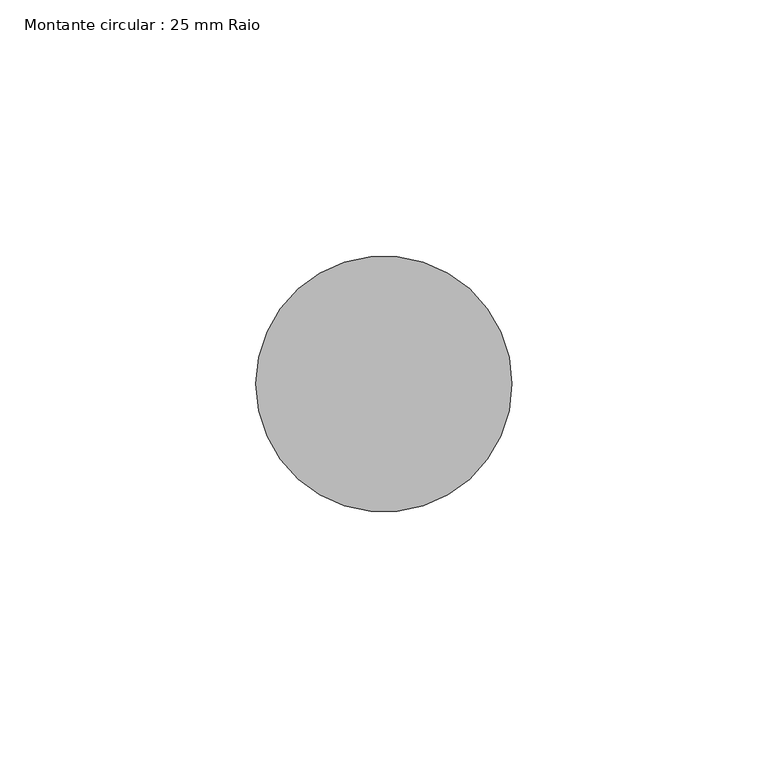
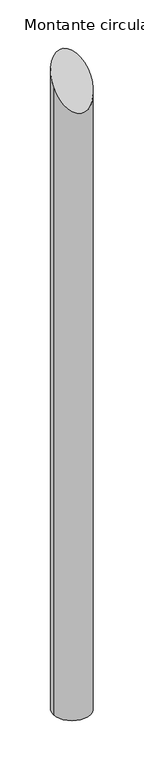
"""IFC4 building model written with IfcOpenShell, lengths in millimetres: member geometry, Montante circular : 25 mm Raio."""

import ifcopenshell
import ifcopenshell.guid

model = None  # the IFC model being written
_history = None  # IfcOwnerHistory: only IFC2X3 demands one
_inside = {}  # id of a spatial element -> (the spatial element, [elements in it])
_under = {}  # id of a project, library or spatial element -> (it, [spatial elements below it])
_declared = {}  # id of a project -> (the project, [libraries it declares])
_typed = {}  # id of a type object -> (the type object, [elements of that type])
_made_of = {}  # id of a material, layer set ... -> (it, [elements and type objects made of it])


def new_model(schema):
    """Start an empty IFC model of exactly this schema.

    Asked for "IFC4X3", IfcOpenShell would pick the latest addendum, in which some entities
    have other attributes; the version numbers below select the first issue.
    IFC2X3 requires an IfcOwnerHistory on every rooted entity: one is made here for all.
    """
    global model, _history
    if schema == "IFC4X3":
        model = ifcopenshell.file(schema_version=(4, 3, 0, 0))
    else:
        model = ifcopenshell.file(schema=schema)
    _inside.clear()
    _under.clear()
    _declared.clear()
    _typed.clear()
    _made_of.clear()
    _history = None
    if model.schema == "IFC2X3":
        org = make("IfcOrganization", Name="unknown")
        user = make(
            "IfcPersonAndOrganization",
            ThePerson=make("IfcPerson", FamilyName="unknown"),
            TheOrganization=org,
        )
        app = make(
            "IfcApplication",
            ApplicationDeveloper=org,
            Version="unknown",
            ApplicationFullName="unknown",
            ApplicationIdentifier="unknown",
        )
        _history = make(
            "IfcOwnerHistory",
            OwningUser=user,
            OwningApplication=app,
            ChangeAction="ADDED",
            CreationDate=0,
        )
    return model


def make(cls, **values):
    """One entity of the class cls with the attributes given. An attribute that is None is left unset."""
    return model.create_entity(
        cls, **{name: value for name, value in values.items() if value is not None}
    )


def rooted(cls, **values):
    """An entity with a GlobalId (a new one), such as an element, a storey or a relation."""
    return make(cls, GlobalId=ifcopenshell.guid.new(), OwnerHistory=_history, **values)


def si_unit(unit_type, name, prefix=None):
    """IfcSIUnit, for example si_unit("LENGTHUNIT", "METRE", prefix="MILLI")."""
    return make("IfcSIUnit", UnitType=unit_type, Prefix=prefix, Name=name)


def assignment(units):
    """IfcUnitAssignment: the units of a project."""
    return None if units is None else make("IfcUnitAssignment", Units=units)


def point(xyz):
    """IfcCartesianPoint."""
    return None if xyz is None else make("IfcCartesianPoint", Coordinates=xyz)


def direction(xyz):
    """IfcDirection."""
    return None if xyz is None else make("IfcDirection", DirectionRatios=xyz)


def frame(location, z_axis=None, x_axis=None):
    """IfcAxis2Placement3D, a coordinate frame: its origin and axes. An axis left out is left unset."""
    return make(
        "IfcAxis2Placement3D",
        Location=point(location),
        Axis=direction(z_axis),
        RefDirection=direction(x_axis),
    )


def origin():
    """The frame at (0, 0, 0) with its axes left unset."""
    return frame((0.0, 0.0, 0.0))


def place(relative_to, where):
    """IfcLocalPlacement: puts the frame where relative to a parent placement (None: the world)."""
    return make(
        "IfcLocalPlacement", PlacementRelTo=relative_to, RelativePlacement=where
    )


def context(
    kind, dimensions, precision=None, world=None, true_north=None, identifier=None
):
    """IfcGeometricRepresentationContext, for example the 3D "Model" context."""
    return make(
        "IfcGeometricRepresentationContext",
        ContextIdentifier=identifier,
        ContextType=kind,
        CoordinateSpaceDimension=dimensions,
        Precision=precision,
        WorldCoordinateSystem=world,
        TrueNorth=true_north,
    )


def project(units=None, contexts=None):
    """IfcProject with its units and contexts."""
    return rooted(
        "IfcProject",
        Name="project",
        RepresentationContexts=contexts,
        UnitsInContext=assignment(units),
    )


def spatial(cls, under=None, at=None, **own):
    """A site, building, storey or space (cls), placed at a placement, below another one or the project."""
    s = rooted(cls, ObjectPlacement=at, **own)
    if under is not None:
        _under.setdefault(under.id(), (under, []))[1].append(s)
    return s


def circle_curve(where, radius):
    """IfcCircle in the frame where."""
    return make("IfcCircle", Position=where, Radius=radius)


def ellipse_curve(where, semi_axis1, semi_axis2):
    """IfcEllipse in the frame where."""
    return make(
        "IfcEllipse", Position=where, SemiAxis1=semi_axis1, SemiAxis2=semi_axis2
    )


def shape(context_of_items, identifier, shape_type, items):
    """IfcShapeRepresentation: the items that make up one representation, for example the "Body"."""
    return make(
        "IfcShapeRepresentation",
        ContextOfItems=context_of_items,
        RepresentationIdentifier=identifier,
        RepresentationType=shape_type,
        Items=items,
    )


def source(mapping_origin, context_of_items, identifier, shape_type, items):
    """IfcRepresentationMap: a shape defined once, which mapped items show again and again."""
    return make(
        "IfcRepresentationMap",
        MappingOrigin=mapping_origin,
        MappedRepresentation=shape(context_of_items, identifier, shape_type, items),
    )


def transform(
    local_origin,
    x_axis=None,
    y_axis=None,
    z_axis=None,
    scale=None,
    scale2=None,
    scale3=None,
    uniform=True,
):
    """IfcCartesianTransformationOperator3D, or its non-uniform kind. x_axis, y_axis, z_axis: its Axis1, 2, 3."""
    if uniform:
        return make(
            "IfcCartesianTransformationOperator3D",
            Axis1=direction(x_axis),
            Axis2=direction(y_axis),
            LocalOrigin=point(local_origin),
            Scale=scale,
            Axis3=direction(z_axis),
        )
    return make(
        "IfcCartesianTransformationOperator3DnonUniform",
        Axis1=direction(x_axis),
        Axis2=direction(y_axis),
        LocalOrigin=point(local_origin),
        Scale=scale,
        Axis3=direction(z_axis),
        Scale2=scale2,
        Scale3=scale3,
    )


def mapped(mapping_source, mapping_target):
    """IfcMappedItem: shows the shape of a source again, moved by a transform."""
    return make(
        "IfcMappedItem", MappingSource=mapping_source, MappingTarget=mapping_target
    )


def made_of(thing, what):
    """Note that an element or type object is made of a material, layer set ...; save() writes the relation."""
    if what is not None:
        _made_of.setdefault(what.id(), (what, []))[1].append(thing)
    return thing


def element(
    cls,
    number,
    at=None,
    inside=None,
    cuts=None,
    type_object=None,
    material=None,
    context=None,
    identifier="Body",
    shape_type=None,
    held_by="IfcProductDefinitionShape",
    body=None,
    shapes=None,
    **own,
):
    """One element of the class cls, such as IfcWall. Its Tag is "e" and its number.

    at: its placement. inside: the storey or other place that contains it. cuts: it is an
    opening in that element (IfcRelVoidsElement). A single representation is given by context,
    identifier, shape_type and body (its items); several are given by shapes. held_by: the class
    of the entity that holds the representations. save() writes the other relations.
    """
    e = rooted(cls, Tag="e%d" % number, ObjectPlacement=at, **own)
    if body is not None:
        shapes = [shape(context, identifier, shape_type, body)]
    if shapes is not None:
        e.Representation = make(held_by, Representations=shapes)
    if inside is not None:
        _inside.setdefault(inside.id(), (inside, []))[1].append(e)
    if cuts is not None:
        rooted(
            "IfcRelVoidsElement", RelatingBuildingElement=cuts, RelatedOpeningElement=e
        )
    if type_object is not None:
        _typed.setdefault(type_object.id(), (type_object, []))[1].append(e)
    return made_of(e, material)


def aggregate(whole, parts):
    """IfcRelAggregates: a whole, such as a stair, and the parts it consists of."""
    return rooted("IfcRelAggregates", RelatingObject=whole, RelatedObjects=parts)


def save(model, path):
    """Write the relations noted so far, then the file.

    IfcRelAggregates (storeys below a building ...), IfcRelContainedInSpatialStructure (elements
    in a storey), IfcRelDefinesByType, IfcRelAssociatesMaterial and IfcRelDeclares: one each for
    every whole, place, type object, material and project.
    """
    for whole, parts in _under.values():
        aggregate(whole, parts)
    for where, things in _inside.values():
        rooted(
            "IfcRelContainedInSpatialStructure",
            RelatedElements=things,
            RelatingStructure=where,
        )
    for kind, things in _typed.values():
        rooted("IfcRelDefinesByType", RelatedObjects=things, RelatingType=kind)
    for what, things in _made_of.values():
        rooted("IfcRelAssociatesMaterial", RelatedObjects=things, RelatingMaterial=what)
    for by, libraries in _declared.values():
        rooted("IfcRelDeclares", RelatingContext=by, RelatedDefinitions=libraries)
    model.write(path)


def plane_surface(at):
    """IfcPlane: the flat surface through the origin of the frame at, square to its z axis."""
    return make("IfcPlane", Position=at)


def cylinder_surface(at, radius):
    """IfcCylindricalSurface: all points at the distance radius from the z axis of the frame at."""
    return make("IfcCylindricalSurface", Position=at, Radius=radius)


def advanced_brep(points, edges, surfaces, faces):
    """IfcAdvancedBrep: a solid bounded by faces that lie on surfaces and meet in shared edges.

    An edge is (start, end): straight between two places in points (the first is 0);
    or (start, end, curve); or (start, end, curve, False) where it runs against its curve.
    A face is (place in surfaces, loops), or (place, loops, False) where it looks against
    its surface's normal. A loop lists edges by number (the first is 1), with a minus sign
    where the edge is run from its end to its start. The first loop is the outer one.
    """
    corners = [point(p) for p in points]
    vertices = [make("IfcVertexPoint", VertexGeometry=c) for c in corners]
    made = []
    for start, end, *more in edges:
        made.append(
            make(
                "IfcEdgeCurve",
                EdgeStart=vertices[start],
                EdgeEnd=vertices[end],
                EdgeGeometry=more[0] if more else make("IfcPolyline", Points=[corners[start], corners[end]]),
                SameSense=more[1] if len(more) > 1 else True,
            )
        )
    hull = []
    for where, loops, *sense in faces:
        bounds = []
        for j, loop in enumerate(loops):
            ring = [make("IfcOrientedEdge", EdgeElement=made[abs(k) - 1], Orientation=k > 0) for k in loop]
            bounds.append(
                make(
                    "IfcFaceOuterBound" if j == 0 else "IfcFaceBound",
                    Bound=make("IfcEdgeLoop", EdgeList=ring),
                    Orientation=True,
                )
            )
        hull.append(make("IfcAdvancedFace", Bounds=bounds, FaceSurface=surfaces[where], SameSense=sense[0] if sense else True))
    return make("IfcAdvancedBrep", Outer=make("IfcClosedShell", CfsFaces=hull))


def montante_circular_25_mm_raio_de2e074c(model_context):
    return source(origin(), model_context, "Body", "AdvancedBrep", [
        advanced_brep(
        [(0.0, 0.0, -893.577346), (-50.0, 0.0, -893.577346), (-50.0, 0.0, 0.0), (0.0, 0.0, 0.0)],
        [
            (0, 1, circle_curve(frame((-25.0, 0.0, -893.577346), z_axis=(0.0, 0.0, -1.0), x_axis=(1.0, 0.0, 0.0)), 25.0)),
            (1, 0, circle_curve(frame((-25.0, 0.0, -893.577346), z_axis=(0.0, 0.0, -1.0), x_axis=(1.0, 0.0, 0.0)), 25.0)),
            (2, 3, ellipse_curve(frame((-25.0, 0.0, 0.0), z_axis=(0.0, 0.7735779641603616, -0.6337011388387355), x_axis=(0.0, 0.6337011388387355, 0.7735779641603616)), 39.4507734, 25.0)),
            (3, 0),
            (1, 2),
            (3, 2, ellipse_curve(frame((-25.0, 0.0, 0.0), z_axis=(0.0, 0.7735779641603616, -0.6337011388387355), x_axis=(0.0, 0.6337011388387355, 0.7735779641603616)), 39.4507734, 25.0)),
        ],
        [
            plane_surface(frame((0.0, -50.0, -893.577346), z_axis=(0.0, 0.0, -1.0), x_axis=(-1.0, 0.0, 0.0))),
            cylinder_surface(frame((-25.0, 0.0, 0.0), z_axis=(0.0, 0.0, 1.0), x_axis=(1.0, 0.0, 0.0)), 25.0),
            plane_surface(frame((304.8, 0.0, 0.0), z_axis=(0.0, -0.7735779641603616, 0.6337011388387355), x_axis=(0.0, -0.6337011388387355, -0.7735779641603616))),
        ],
        [
            (0, [[1, 2]]),
            (1, [[3, 4, -2, 5]]),
            (1, [[6, -5, -1, -4]]),
            (2, [[-3, -6]]),
        ],
    ),
    ])


if __name__ == "__main__":
    model = new_model("IFC4")
    model_context = context("Model", 3, world=origin())
    ifc_project = project(units=[si_unit("LENGTHUNIT", "METRE", prefix="MILLI")], contexts=[model_context])
    site = spatial("IfcSite", under=ifc_project)
    building = spatial("IfcBuilding", under=site)
    placement = place(None, origin())
    montante_circular_25_mm_raio_shape = montante_circular_25_mm_raio_de2e074c(model_context)
    element("IfcMember", 1, ObjectType="Montante circular : 25 mm Raio", at=placement, inside=building, context=model_context, shape_type="MappedRepresentation", body=[
        mapped(montante_circular_25_mm_raio_shape, transform((0.0, 0.0, 0.0), x_axis=(1.0, 0.0, 0.0), y_axis=(0.0, 1.0, 0.0), z_axis=(0.0, 0.0, 1.0))),
    ])
    save(model, "model.ifc")

# Revit data of these elements
# Type "Montante circular : 25 mm Raio"
#   built-in parameter 1007350 = 0.082021 (stored number, unit not read)
# Element 1 (IfcMember, "Montante circular : 25 mm Raio")
#   Materials on its faces: "Alumín."
# Materials
#   "Alumín.": class "Metal", colour RGB 247 247 247, transparency 0, Description = "Alumín. 6061", Cost = 0
